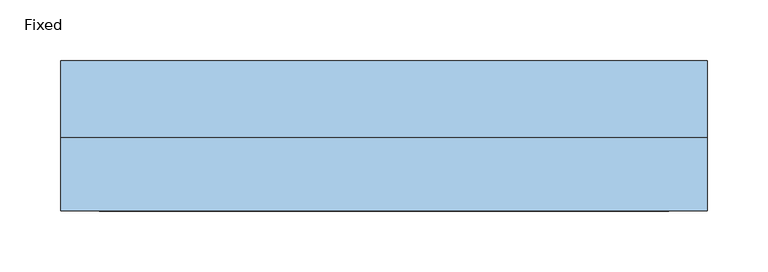
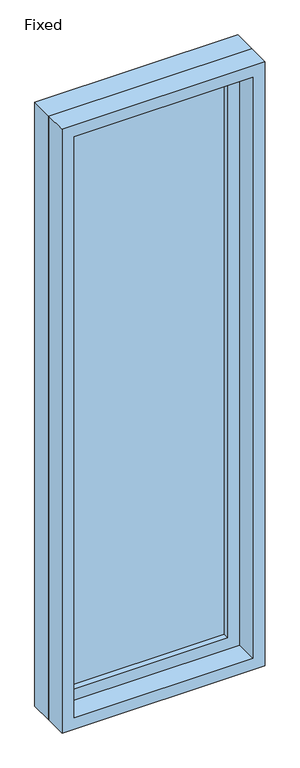
"""IFC4 building model written with IfcOpenShell, lengths in millimetres: window geometry, Fixed."""

from ifc_helpers import new_model, si_unit, frame, origin, place, context, project, spatial, polyline, outline, extrude, source, transform, mapped, element, save


def fixed_82522c54(model_context):
    return source(origin(), model_context, "Body", "SweptSolid", [
        extrude(outline(polyline([(165.1, 14.2875), (-241.3, 14.2875), (-241.3, 26.9875), (165.1, 26.9875), (165.1, 14.2875)])), frame((0.0, 0.0, 825.5), z_axis=(0.0, 0.0, 1.0), x_axis=(1.0, 0.0, 0.0)), (0.0, 0.0, 1.0), 1549.4),
        extrude(outline(polyline([(2419.35, -285.75), (781.05, -285.75), (781.05, 209.55), (2419.35, 209.55), (2419.35, -285.75)]), holes=[polyline([(2374.9, -241.3), (2374.9, 165.1), (825.5, 165.1), (825.5, -241.3), (2374.9, -241.3)])]), frame((0.0, -1.5875, 0.0), z_axis=(0.0, 1.0, 0.0), x_axis=(0.0, 0.0, 1.0)), (0.0, 0.0, 1.0), 44.45),
        extrude(outline(polyline([(2438.4, -304.8), (762.0, -304.8), (762.0, 228.6), (2438.4, 228.6), (2438.4, -304.8)]), holes=[polyline([(2406.65, -273.05), (2406.65, 196.85), (793.75, 196.85), (793.75, -273.05), (2406.65, -273.05)])]), frame((0.0, -61.9125, 0.0), z_axis=(0.0, 1.0, 0.0), x_axis=(0.0, 0.0, 1.0)), (0.0, 0.0, 1.0), 60.325),
        extrude(outline(polyline([(2438.4, 228.6), (2438.4, -304.8), (762.0, -304.8), (762.0, 228.6), (2438.4, 228.6)]), holes=[polyline([(2419.35, 209.55), (781.05, 209.55), (781.05, -285.75), (2419.35, -285.75), (2419.35, 209.55)])]), frame((0.0, -1.5875, 0.0), z_axis=(0.0, 1.0, 0.0), x_axis=(0.0, 0.0, 1.0)), (0.0, 0.0, 1.0), 63.5),
    ])


if __name__ == "__main__":
    model = new_model("IFC4")
    model_context = context("Model", 3, world=origin())
    ifc_project = project(units=[si_unit("LENGTHUNIT", "METRE", prefix="MILLI")], contexts=[model_context])
    site = spatial("IfcSite", under=ifc_project)
    building = spatial("IfcBuilding", under=site)
    placement = place(None, origin())
    fixed_shape = fixed_82522c54(model_context)
    element("IfcWindow", 1, ObjectType="Fixed : 66\" x 21\"  Screen", at=placement, inside=building, context=model_context, shape_type="MappedRepresentation", body=[
        mapped(fixed_shape, transform((0.0, 0.0, 0.0), x_axis=(1.0, 0.0, 0.0), y_axis=(0.0, 1.0, 0.0), z_axis=(0.0, 0.0, 1.0))),
    ])
    save(model, "model.ifc")

# Revit data of these elements
# Type "Fixed : 66\" x 21\"  Screen"
#   Type Mark = "70"
#   COBie.Type.CreatedBy = "doug.wood@us.ibm.com"
#   COBie.Type.CreatedOn = "2016-04-14T02:07:26"
#   COBie.Type.Name = "Windows_Fixed_66\" x 21\"  Screen_70"
#   COBie.Type.Category = "23-30 20 17 11 : Fixed Windows"
#   COBie.Type.Description = "Fixed_66\" x 21\"  Screen"
#   COBie.Type.Manufacturer = ""
#   COBie.Type.ModelNumber = ""
#   Construction Type Id = "GSP4R"
#   Assembly Code = "B2020100"
#   Analytic Construction = "1/8 in Pilkington single glazing"
#   COBie.Type.ReplacementCost = 0
#   Visual Light Transmittance = 0.9
#   Solar Heat Gain Coefficient = 0.78
#   Heat Transfer Coefficient (U) = 3.6886 W/(m²·K)
#   Height = 5' - 6"
#   Default Sill Height = 2' - 6"
#   Width = 1' - 9"
#   Window Inset = 0' - 0 3/4"
#   COBie.Type = no
#   Glass Pane Material = Screen
#   Sash Material = Sash - White
#   Wall Closure = (empty or 0)
# Element 1 (IfcWindow, "Fixed : 66\" x 21\"  Screen")
#   Materials on its faces: "Sash - White", "Screen"
# Materials
#   "Screen": class "Metal", colour RGB 120 120 120, transparency 0, Description = "Screen", Cost = 0
#   "Sash - White": class "Wood", colour RGB 255 255 255, transparency 0, Cost = 0
